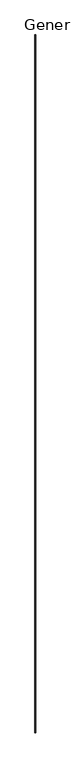
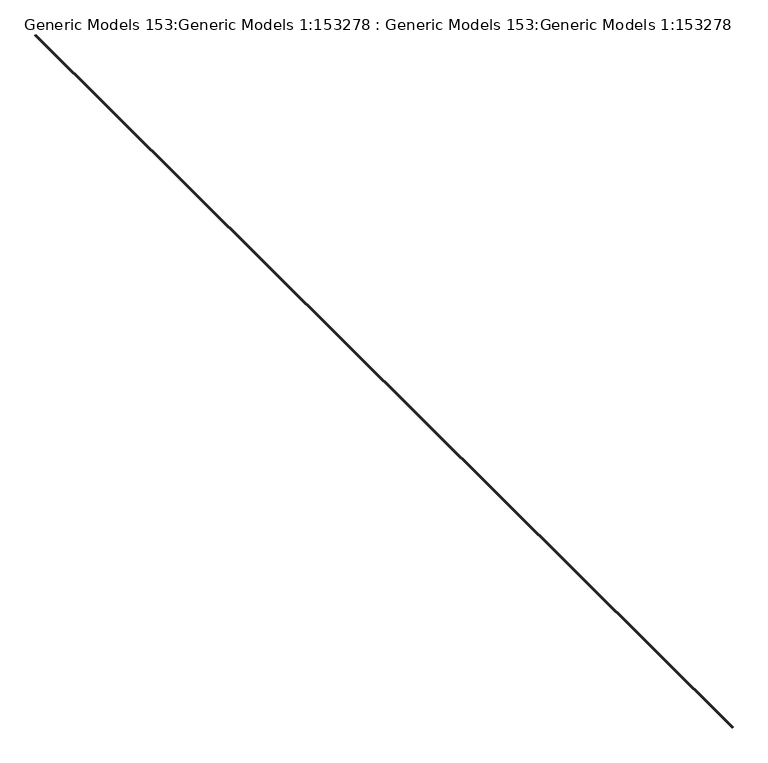
"""IFC4 building model written with IfcOpenShell, lengths in millimetres: proxy geometry, Generic Models 153:Generic Models 1:153278 : Generic Models 153:Generic Models 1:153278."""

import ifcopenshell
import ifcopenshell.guid

model = None  # the IFC model being written
_history = None  # IfcOwnerHistory: only IFC2X3 demands one
_inside = {}  # id of a spatial element -> (the spatial element, [elements in it])
_under = {}  # id of a project, library or spatial element -> (it, [spatial elements below it])
_declared = {}  # id of a project -> (the project, [libraries it declares])
_typed = {}  # id of a type object -> (the type object, [elements of that type])
_made_of = {}  # id of a material, layer set ... -> (it, [elements and type objects made of it])


def new_model(schema):
    """Start an empty IFC model of exactly this schema.

    Asked for "IFC4X3", IfcOpenShell would pick the latest addendum, in which some entities
    have other attributes; the version numbers below select the first issue.
    IFC2X3 requires an IfcOwnerHistory on every rooted entity: one is made here for all.
    """
    global model, _history
    if schema == "IFC4X3":
        model = ifcopenshell.file(schema_version=(4, 3, 0, 0))
    else:
        model = ifcopenshell.file(schema=schema)
    _inside.clear()
    _under.clear()
    _declared.clear()
    _typed.clear()
    _made_of.clear()
    _history = None
    if model.schema == "IFC2X3":
        org = make("IfcOrganization", Name="unknown")
        user = make(
            "IfcPersonAndOrganization",
            ThePerson=make("IfcPerson", FamilyName="unknown"),
            TheOrganization=org,
        )
        app = make(
            "IfcApplication",
            ApplicationDeveloper=org,
            Version="unknown",
            ApplicationFullName="unknown",
            ApplicationIdentifier="unknown",
        )
        _history = make(
            "IfcOwnerHistory",
            OwningUser=user,
            OwningApplication=app,
            ChangeAction="ADDED",
            CreationDate=0,
        )
    return model


def make(cls, **values):
    """One entity of the class cls with the attributes given. An attribute that is None is left unset."""
    return model.create_entity(
        cls, **{name: value for name, value in values.items() if value is not None}
    )


def rooted(cls, **values):
    """An entity with a GlobalId (a new one), such as an element, a storey or a relation."""
    return make(cls, GlobalId=ifcopenshell.guid.new(), OwnerHistory=_history, **values)


def si_unit(unit_type, name, prefix=None):
    """IfcSIUnit, for example si_unit("LENGTHUNIT", "METRE", prefix="MILLI")."""
    return make("IfcSIUnit", UnitType=unit_type, Prefix=prefix, Name=name)


def assignment(units):
    """IfcUnitAssignment: the units of a project."""
    return None if units is None else make("IfcUnitAssignment", Units=units)


def point(xyz):
    """IfcCartesianPoint."""
    return None if xyz is None else make("IfcCartesianPoint", Coordinates=xyz)


def direction(xyz):
    """IfcDirection."""
    return None if xyz is None else make("IfcDirection", DirectionRatios=xyz)


def frame(location, z_axis=None, x_axis=None):
    """IfcAxis2Placement3D, a coordinate frame: its origin and axes. An axis left out is left unset."""
    return make(
        "IfcAxis2Placement3D",
        Location=point(location),
        Axis=direction(z_axis),
        RefDirection=direction(x_axis),
    )


def frame_2d(location, x_axis=None):
    """IfcAxis2Placement2D, a coordinate frame in the plane: its origin and x axis."""
    return make(
        "IfcAxis2Placement2D", Location=point(location), RefDirection=direction(x_axis)
    )


def origin():
    """The frame at (0, 0, 0) with its axes left unset."""
    return frame((0.0, 0.0, 0.0))


def place(relative_to, where):
    """IfcLocalPlacement: puts the frame where relative to a parent placement (None: the world)."""
    return make(
        "IfcLocalPlacement", PlacementRelTo=relative_to, RelativePlacement=where
    )


def context(
    kind, dimensions, precision=None, world=None, true_north=None, identifier=None
):
    """IfcGeometricRepresentationContext, for example the 3D "Model" context."""
    return make(
        "IfcGeometricRepresentationContext",
        ContextIdentifier=identifier,
        ContextType=kind,
        CoordinateSpaceDimension=dimensions,
        Precision=precision,
        WorldCoordinateSystem=world,
        TrueNorth=true_north,
    )


def project(units=None, contexts=None):
    """IfcProject with its units and contexts."""
    return rooted(
        "IfcProject",
        Name="project",
        RepresentationContexts=contexts,
        UnitsInContext=assignment(units),
    )


def spatial(cls, under=None, at=None, **own):
    """A site, building, storey or space (cls), placed at a placement, below another one or the project."""
    s = rooted(cls, ObjectPlacement=at, **own)
    if under is not None:
        _under.setdefault(under.id(), (under, []))[1].append(s)
    return s


def polyline(points):
    """IfcPolyline through the points."""
    return make("IfcPolyline", Points=[point(p) for p in points])


def circle_curve(where, radius):
    """IfcCircle in the frame where."""
    return make("IfcCircle", Position=where, Radius=radius)


def trimmed(basis, trim1, trim2, sense, master):
    """IfcTrimmedCurve: the piece of a basis curve between two trims."""
    return make(
        "IfcTrimmedCurve",
        BasisCurve=basis,
        Trim1=trim1,
        Trim2=trim2,
        SenseAgreement=sense,
        MasterRepresentation=master,
    )


def segment(curve, same_sense, transition):
    """IfcCompositeCurveSegment."""
    return make(
        "IfcCompositeCurveSegment",
        Transition=transition,
        SameSense=same_sense,
        ParentCurve=curve,
    )


def composite_curve(segments, self_intersect=None):
    """IfcCompositeCurve: segments joined end to end."""
    return make("IfcCompositeCurve", Segments=segments, SelfIntersect=self_intersect)


def outline(outer, holes=None, kind="AREA"):
    """IfcArbitraryClosedProfileDef: a profile drawn as a closed curve; with holes, ...WithVoids."""
    if holes is None:
        return make("IfcArbitraryClosedProfileDef", ProfileType=kind, OuterCurve=outer)
    return make(
        "IfcArbitraryProfileDefWithVoids",
        ProfileType=kind,
        OuterCurve=outer,
        InnerCurves=holes,
    )


def extrude(swept, where, along, depth):
    """IfcExtrudedAreaSolid: the profile swept, set in the frame where, extruded along a direction by depth."""
    return make(
        "IfcExtrudedAreaSolid",
        SweptArea=swept,
        Position=where,
        ExtrudedDirection=direction(along),
        Depth=depth,
    )


def shape(context_of_items, identifier, shape_type, items):
    """IfcShapeRepresentation: the items that make up one representation, for example the "Body"."""
    return make(
        "IfcShapeRepresentation",
        ContextOfItems=context_of_items,
        RepresentationIdentifier=identifier,
        RepresentationType=shape_type,
        Items=items,
    )


def source(mapping_origin, context_of_items, identifier, shape_type, items):
    """IfcRepresentationMap: a shape defined once, which mapped items show again and again."""
    return make(
        "IfcRepresentationMap",
        MappingOrigin=mapping_origin,
        MappedRepresentation=shape(context_of_items, identifier, shape_type, items),
    )


def transform(
    local_origin,
    x_axis=None,
    y_axis=None,
    z_axis=None,
    scale=None,
    scale2=None,
    scale3=None,
    uniform=True,
):
    """IfcCartesianTransformationOperator3D, or its non-uniform kind. x_axis, y_axis, z_axis: its Axis1, 2, 3."""
    if uniform:
        return make(
            "IfcCartesianTransformationOperator3D",
            Axis1=direction(x_axis),
            Axis2=direction(y_axis),
            LocalOrigin=point(local_origin),
            Scale=scale,
            Axis3=direction(z_axis),
        )
    return make(
        "IfcCartesianTransformationOperator3DnonUniform",
        Axis1=direction(x_axis),
        Axis2=direction(y_axis),
        LocalOrigin=point(local_origin),
        Scale=scale,
        Axis3=direction(z_axis),
        Scale2=scale2,
        Scale3=scale3,
    )


def mapped(mapping_source, mapping_target):
    """IfcMappedItem: shows the shape of a source again, moved by a transform."""
    return make(
        "IfcMappedItem", MappingSource=mapping_source, MappingTarget=mapping_target
    )


def made_of(thing, what):
    """Note that an element or type object is made of a material, layer set ...; save() writes the relation."""
    if what is not None:
        _made_of.setdefault(what.id(), (what, []))[1].append(thing)
    return thing


def element(
    cls,
    number,
    at=None,
    inside=None,
    cuts=None,
    type_object=None,
    material=None,
    context=None,
    identifier="Body",
    shape_type=None,
    held_by="IfcProductDefinitionShape",
    body=None,
    shapes=None,
    **own,
):
    """One element of the class cls, such as IfcWall. Its Tag is "e" and its number.

    at: its placement. inside: the storey or other place that contains it. cuts: it is an
    opening in that element (IfcRelVoidsElement). A single representation is given by context,
    identifier, shape_type and body (its items); several are given by shapes. held_by: the class
    of the entity that holds the representations. save() writes the other relations.
    """
    e = rooted(cls, Tag="e%d" % number, ObjectPlacement=at, **own)
    if body is not None:
        shapes = [shape(context, identifier, shape_type, body)]
    if shapes is not None:
        e.Representation = make(held_by, Representations=shapes)
    if inside is not None:
        _inside.setdefault(inside.id(), (inside, []))[1].append(e)
    if cuts is not None:
        rooted(
            "IfcRelVoidsElement", RelatingBuildingElement=cuts, RelatedOpeningElement=e
        )
    if type_object is not None:
        _typed.setdefault(type_object.id(), (type_object, []))[1].append(e)
    return made_of(e, material)


def aggregate(whole, parts):
    """IfcRelAggregates: a whole, such as a stair, and the parts it consists of."""
    return rooted("IfcRelAggregates", RelatingObject=whole, RelatedObjects=parts)


def save(model, path):
    """Write the relations noted so far, then the file.

    IfcRelAggregates (storeys below a building ...), IfcRelContainedInSpatialStructure (elements
    in a storey), IfcRelDefinesByType, IfcRelAssociatesMaterial and IfcRelDeclares: one each for
    every whole, place, type object, material and project.
    """
    for whole, parts in _under.values():
        aggregate(whole, parts)
    for where, things in _inside.values():
        rooted(
            "IfcRelContainedInSpatialStructure",
            RelatedElements=things,
            RelatingStructure=where,
        )
    for kind, things in _typed.values():
        rooted("IfcRelDefinesByType", RelatedObjects=things, RelatingType=kind)
    for what, things in _made_of.values():
        rooted("IfcRelAssociatesMaterial", RelatedObjects=things, RelatingMaterial=what)
    for by, libraries in _declared.values():
        rooted("IfcRelDeclares", RelatingContext=by, RelatedDefinitions=libraries)
    model.write(path)


def generic_models_153_generic_models_1_153278_generic_models_26376bb5(model_context):
    return source(origin(), model_context, "Body", "SweptSolid", [
        extrude(outline(composite_curve([segment(polyline([(2885.8668287, -6544.8418716), (2885.8668287, -6540.0793716)]), True, "CONTINUOUS"), segment(trimmed(circle_curve(frame_2d((2890.6293287, -6535.7072608)), 6.4650413), [point((2885.8668287, -6540.0793716))], [point((2895.3918287, -6540.0793716))], True, "CARTESIAN"), True, "CONTINUOUS"), segment(polyline([(2895.3918287, -6540.0793716), (2895.3918287, -6544.8418716)]), True, "CONTINUOUS"), segment(trimmed(circle_curve(frame_2d((2890.6293287, -6540.4697608)), 6.4650413), [point((2895.3918287, -6544.8418716))], [point((2893.4858409, -6546.2695105))], False, "CARTESIAN"), True, "CONTINUOUS"), segment(polyline([(2893.4858409, -6546.2695105), (2894.2400753, -6547.3274234), (2894.8245637, -6548.6043243), (2895.2118287, -6550.0401844), (2895.3836643, -6551.567502), (2895.3319923, -6553.114476), (2895.059242, -6554.6083811), (2894.5782356, -6555.9789868), (2893.9115859, -6557.1618592), (2893.0906331, -6558.1013898), (2892.153971, -6558.7534101), (2891.1456335, -6559.0872678), (2890.1130239, -6559.0872678), (2889.1046864, -6558.7534101), (2888.1680244, -6558.1013898), (2887.3470715, -6557.1618592), (2886.6804218, -6555.9789868), (2886.1994154, -6554.6083811), (2885.9266651, -6553.114476), (2885.8749931, -6551.567502), (2886.0468287, -6550.0401844), (2886.4340937, -6548.6043243), (2887.0185822, -6547.3274234), (2887.7728165, -6546.2695105)]), True, "CONTINUOUS"), segment(trimmed(circle_curve(frame_2d((2890.6293287, -6540.4697608)), 6.4650413), [point((2887.7728165, -6546.2695105))], [point((2885.8668287, -6544.8418716))], False, "CARTESIAN"), True, "CONTINUOUS")], self_intersect=False)), frame((0.0, -6877.9974793, 0.0), z_axis=(0.0, 1.0, 0.0), x_axis=(0.0, 0.0, 1.0)), (0.0, 0.0, 1.0), 19050.0),
    ])


if __name__ == "__main__":
    model = new_model("IFC4")
    model_context = context("Model", 3, world=origin())
    ifc_project = project(units=[si_unit("LENGTHUNIT", "METRE", prefix="MILLI")], contexts=[model_context])
    site = spatial("IfcSite", under=ifc_project)
    building = spatial("IfcBuilding", under=site)
    placement = place(None, origin())
    generic_models_153_generic_models_1_153278_generic_models_shape = generic_models_153_generic_models_1_153278_generic_models_26376bb5(model_context)
    element("IfcBuildingElementProxy", 1, Name="Generic Models 153:Generic Models 1:153278 : Generic Models 153:Generic Models 1:153278", ObjectType="Generic Models 153:Generic Models 1:153278 : Generic Models 153:Generic Models 1:153278", at=placement, inside=building, context=model_context, shape_type="MappedRepresentation", body=[
        mapped(generic_models_153_generic_models_1_153278_generic_models_shape, transform((0.0, 0.0, 0.0), x_axis=(1.0, 0.0, 0.0), y_axis=(0.0, 1.0, 0.0), z_axis=(0.0, 0.0, 1.0))),
    ])
    save(model, "model.ifc")

# Revit data of these elements
# Type "Generic Models 153:Generic Models 1:153278 : Generic Models 153:Generic Models 1:153278"
#   NameOverride = "Generic Models 153:Generic Models 1:153278"
#   ObjectTypeOverride = "Generic Models 153:Generic Models 1"
#   Reference = "Generic Models 1"
#   Category = "Generic Models"
#   Tag = "153278"
# Element 1 (IfcBuildingElementProxy, "Generic Models 153:Generic Models 1:153278 : Generic Models 153:Generic Models 1:153278")
#   Materials on its faces: "_SEALANT AND BACKROD, IF NECESSARY 12051"
# Materials
#   "_SEALANT AND BACKROD, IF NECESSARY 12051": class "Unassigned", colour RGB 190 220 196, transparency 0
